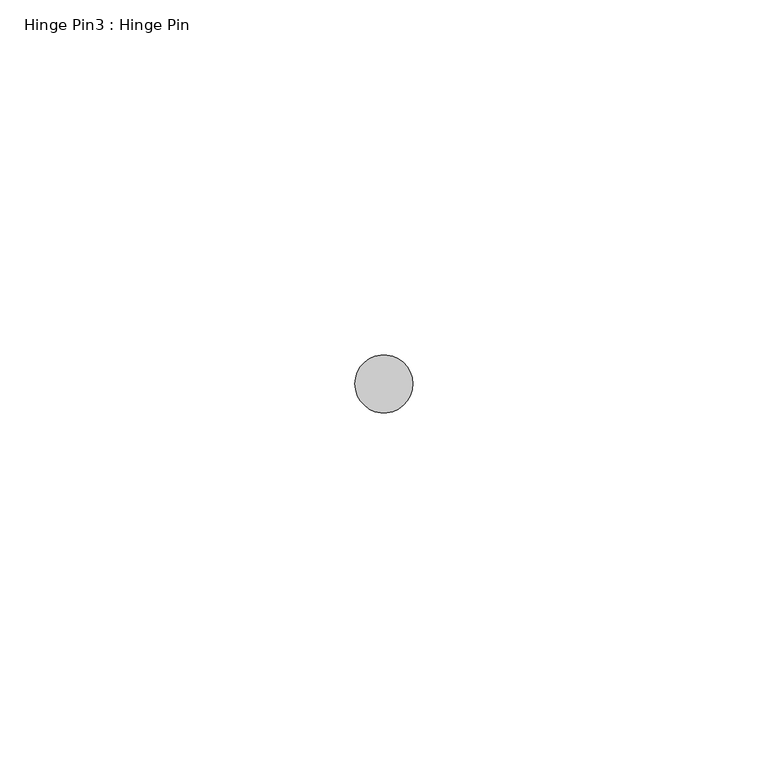
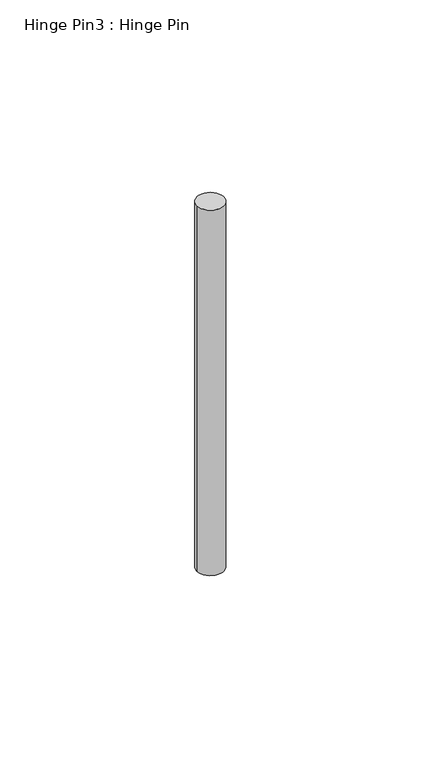
"""IFC4 building model written with IfcOpenShell, lengths in millimetres: proxy geometry, Hinge Pin3 : Hinge Pin."""

from ifc_helpers import new_model, si_unit, point, frame, frame_2d, origin, place, context, project, spatial, circle_curve, trimmed, segment, composite_curve, outline, extrude, source, transform, mapped, element, save


def hinge_pin3_hinge_pin_7876437f(model_context):
    return source(origin(), model_context, "Body", "SweptSolid", [
        extrude(outline(composite_curve([segment(trimmed(circle_curve(frame_2d((587319.1320739, -533984.6777841)), 4.0894), [point((587315.0426739, -533984.6777841))], [point((587323.2214739, -533984.6777841))], False, "CARTESIAN"), True, "CONTINUOUS"), segment(trimmed(circle_curve(frame_2d((587319.1320739, -533984.6777841)), 4.0894), [point((587323.2214739, -533984.6777841))], [point((587315.0426739, -533984.6777841))], False, "CARTESIAN"), True, "CONTINUOUS")], self_intersect=False)), frame((0.0, 0.0, 1941.3140625), z_axis=(0.0, 0.0, 1.0), x_axis=(1.0, 0.0, 0.0)), (0.0, 0.0, 1.0), 117.871875),
    ])


if __name__ == "__main__":
    model = new_model("IFC4")
    model_context = context("Model", 3, world=origin())
    ifc_project = project(units=[si_unit("LENGTHUNIT", "METRE", prefix="MILLI")], contexts=[model_context])
    site = spatial("IfcSite", under=ifc_project)
    building = spatial("IfcBuilding", under=site)
    placement = place(None, origin())
    hinge_pin3_hinge_pin_shape = hinge_pin3_hinge_pin_7876437f(model_context)
    element("IfcBuildingElementProxy", 1, Name="Hinge Pin3 : Hinge Pin", ObjectType="Hinge Pin3 : Hinge Pin", at=placement, inside=building, context=model_context, shape_type="MappedRepresentation", body=[
        mapped(hinge_pin3_hinge_pin_shape, transform((0.0, 0.0, 0.0), x_axis=(1.0, 0.0, 0.0), y_axis=(0.0, 1.0, 0.0), z_axis=(0.0, 0.0, 1.0))),
    ])
    save(model, "model.ifc")

# Revit data of these elements
# Element 1 (IfcBuildingElementProxy, "Hinge Pin3 : Hinge Pin")
#   Materials on its faces: "6\"X6\" WELD-ON STL BUTT HINGE"
# Materials
#   "6\"X6\" WELD-ON STL BUTT HINGE": class "Metal", colour RGB 189 187 185, transparency 0, Description = "Carbon steel", Cost = 0
